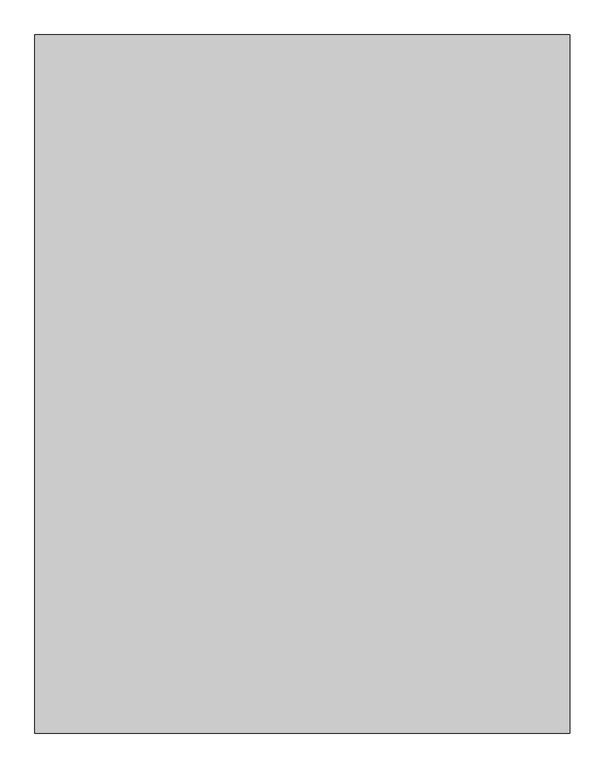
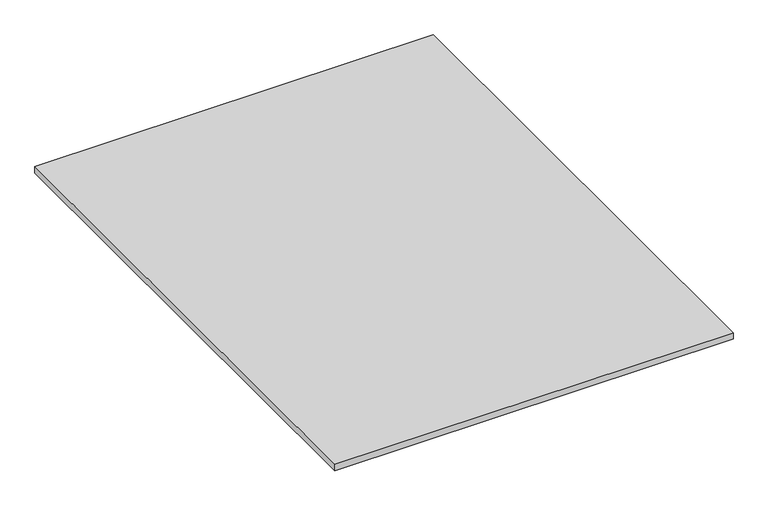
"""IFC4 building model written with IfcOpenShell, lengths in millimetres: proxy geometry, Soffit003 936 : Soffit003 936."""

from ifc_helpers import new_model, si_unit, frame, origin, place, context, project, spatial, polyline, outline, extrude, source, transform, mapped, element, save


def generic_models_0a5e932d(model_context):
    return source(origin(), model_context, "Body", "SweptSolid", [
        extrude(outline(polyline([(-4952.2707965, 7982.1531721), (-6484.1211227, 7982.1531721), (-6484.1211227, 9982.1531721), (-4952.2707965, 9982.1531721), (-4952.2707965, 7982.1531721)])), frame((0.0, 0.0, 43030.1617235), z_axis=(0.0, 0.0, 1.0), x_axis=(1.0, 0.0, 0.0)), (0.0, 0.0, 1.0), 26.0465759),
    ])


if __name__ == "__main__":
    model = new_model("IFC4")
    model_context = context("Model", 3, world=origin())
    ifc_project = project(units=[si_unit("LENGTHUNIT", "METRE", prefix="MILLI")], contexts=[model_context])
    site = spatial("IfcSite", under=ifc_project)
    building = spatial("IfcBuilding", under=site)
    placement = place(None, origin())
    generic_models_shape = generic_models_0a5e932d(model_context)
    element("IfcBuildingElementProxy", 1, Name="Soffit003 936 : Soffit003 936", ObjectType="Soffit003 936 : Soffit003 936", at=placement, inside=building, context=model_context, shape_type="MappedRepresentation", body=[
        mapped(generic_models_shape, transform((0.0, 0.0, 0.0), x_axis=(1.0, 0.0, 0.0), y_axis=(0.0, 1.0, 0.0), z_axis=(0.0, 0.0, 1.0))),
    ])
    save(model, "model.ifc")

# Revit data of these elements
# Type "Soffit003 936 : Soffit003 936"
#   NameOverride = "Soffit003"
# Element 1 (IfcBuildingElementProxy, "Soffit003 936 : Soffit003 936")
#   Materials on its faces: "WHITE OAK OVER BUILDING WRAP"
# Materials
#   "WHITE OAK OVER BUILDING WRAP": class "Unassigned", colour RGB 227 188 136, transparency 0, Cost = 0
